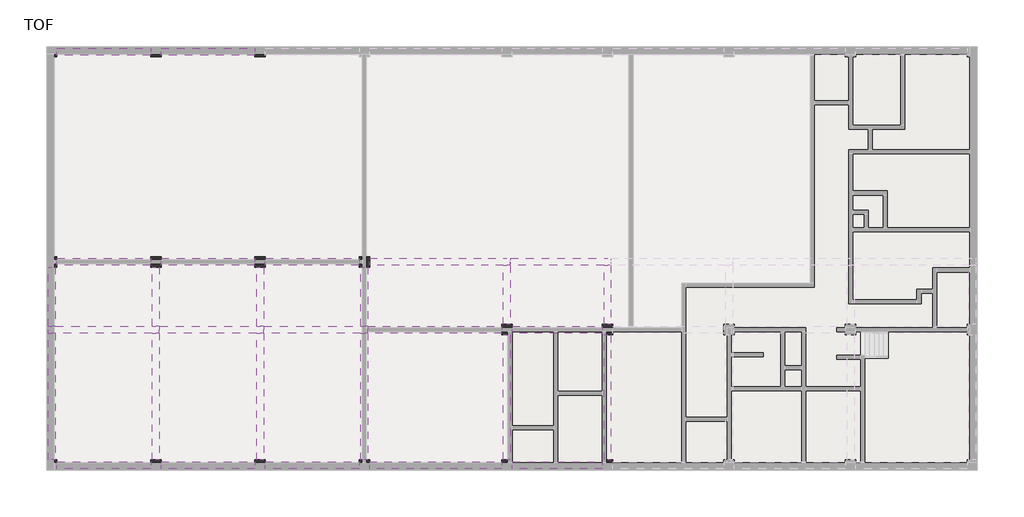
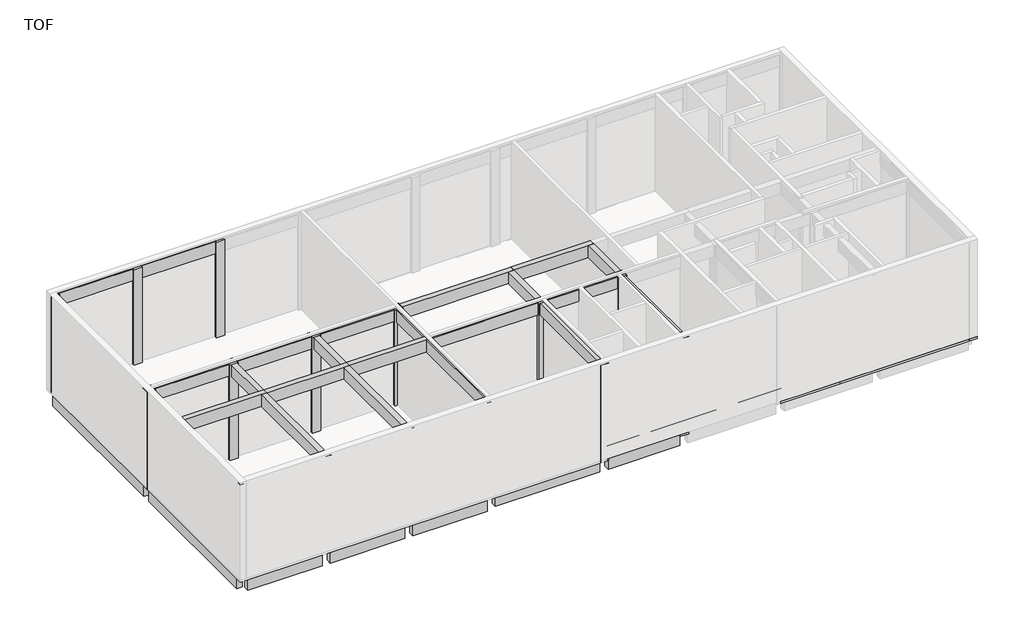
# One storey, part 2 of 3: 38 beams, 15 columns, 4 slabs.
"""IFC4 building model written with IfcOpenShell, lengths in millimetres."""

from ifc_helpers import new_model, si_unit, frame, origin, origin_with_axes, place, context, project, spatial, polyline, outline, extrude, faceted_brep, element, save

model = new_model("IFC4")

# Units and contexts
model_context = context("Model", 3, world=origin())
ifc_project = project(units=[si_unit("LENGTHUNIT", "METRE", prefix="MILLI")], contexts=[model_context])

# Site, building, storey
site = spatial("IfcSite", under=ifc_project)
building = spatial("IfcBuilding", under=site)
storey = spatial("IfcBuildingStorey", under=building, Name="TOF", Elevation=150.0)

# Beams
placement = place(None, origin())
element("IfcBeam", 1, ObjectType="RC Beam_Rectangular : H_SB_ACB_B400xH900", at=placement, inside=storey, context=model_context, shape_type="SweptSolid", body=[
    extrude(outline(polyline([(124.7, 12616.5208589), (-275.3, 12616.5208589), (-275.3, 24116.5208589), (124.7, 24116.5208589), (124.7, 12616.5208589)])), frame((0.0, 0.0, -900.0), z_axis=(0.0, 0.0, 1.0), x_axis=(1.0, 0.0, 0.0)), (0.0, 0.0, 1.0), 900.0),
])
element("IfcBeam", 2, ObjectType="RC Beam_Rectangular : H_SB_ACB_B400xH900", at=placement, inside=storey, context=model_context, shape_type="SweptSolid", body=[
    extrude(outline(polyline([(124.7, 916.5208589), (-275.3, 916.5208589), (-275.3, 12016.5208589), (124.7, 12016.5208589), (124.7, 916.5208589)])), frame((0.0, 0.0, -900.0), z_axis=(0.0, 0.0, 1.0), x_axis=(1.0, 0.0, 0.0)), (0.0, 0.0, 1.0), 900.0),
])
element("IfcBeam", 3, ObjectType="RC Beam_Rectangular : H_SB_ACB_B400xH900", at=placement, inside=storey, context=model_context, shape_type="SweptSolid", body=[
    extrude(outline(polyline([(5624.7, 24616.5208589), (5624.7, 24216.5208589), (224.7, 24216.5208589), (224.7, 24616.5208589), (5624.7, 24616.5208589)])), frame((0.0, 0.0, -900.0), z_axis=(0.0, 0.0, 1.0), x_axis=(1.0, 0.0, 0.0)), (0.0, 0.0, 1.0), 900.0),
])
element("IfcBeam", 4, ObjectType="RC Beam_Rectangular : H_SB_ACB_B400xH900", at=placement, inside=storey, context=model_context, shape_type="SweptSolid", body=[
    extrude(outline(polyline([(6224.7, 24216.5208589), (6224.7, 24616.5208589), (11624.7, 24616.5208589), (11624.7, 24216.5208589), (6224.7, 24216.5208589)])), frame((0.0, 0.0, -900.0), z_axis=(0.0, 0.0, 1.0), x_axis=(1.0, 0.0, 0.0)), (0.0, 0.0, 1.0), 900.0),
])
element("IfcBeam", 5, ObjectType="RC Beam_Rectangular : H_SB_ACB_B400xH900", at=placement, inside=storey, context=model_context, shape_type="SweptSolid", body=[
    extrude(outline(polyline([(224.7, 416.5208589), (224.7, 816.5208589), (5624.7, 816.5208589), (5624.7, 416.5208589), (224.7, 416.5208589)])), frame((0.0, 0.0, -900.0), z_axis=(0.0, 0.0, 1.0), x_axis=(1.0, 0.0, 0.0)), (0.0, 0.0, 1.0), 900.0),
])
element("IfcBeam", 6, ObjectType="RC Beam_Rectangular : H_SB_ACB_B400xH900", at=placement, inside=storey, context=model_context, shape_type="SweptSolid", body=[
    extrude(outline(polyline([(6224.7, 416.5208589), (6224.7, 816.5208589), (11624.7, 816.5208589), (11624.7, 416.5208589), (6224.7, 416.5208589)])), frame((0.0, 0.0, -900.0), z_axis=(0.0, 0.0, 1.0), x_axis=(1.0, 0.0, 0.0)), (0.0, 0.0, 1.0), 900.0),
])
element("IfcBeam", 7, ObjectType="RC Beam_Rectangular : H_SB_ACB_B400xH900", at=placement, inside=storey, context=model_context, shape_type="SweptSolid", body=[
    extrude(outline(polyline([(12224.7, 416.5208589), (12224.7, 816.5208589), (17624.7, 816.5208589), (17624.7, 416.5208589), (12224.7, 416.5208589)])), frame((0.0, 0.0, -900.0), z_axis=(0.0, 0.0, 1.0), x_axis=(1.0, 0.0, 0.0)), (0.0, 0.0, 1.0), 900.0),
])
element("IfcBeam", 8, ObjectType="RC Beam_Rectangular : H_SB_ACB_B400xH900", at=placement, inside=storey, context=model_context, shape_type="SweptSolid", body=[
    extrude(outline(polyline([(18224.7, 416.5208589), (18224.7, 816.5208589), (25824.7, 816.5208589), (25824.7, 416.5208589), (18224.7, 416.5208589)])), frame((0.0, 0.0, -750.0), z_axis=(0.0, 0.0, 1.0), x_axis=(1.0, 0.0, 0.0)), (0.0, 0.0, 1.0), 900.0),
])
element("IfcBeam", 9, ObjectType="RC Beam_Rectangular : H_SB_ACB_B400xH900", at=placement, inside=storey, context=model_context, shape_type="SweptSolid", body=[
    extrude(outline(polyline([(26424.7, 416.5208589), (26424.7, 816.5208589), (31624.7, 816.5208589), (31624.7, 416.5208589), (26424.7, 416.5208589)])), frame((0.0, 0.0, -750.0), z_axis=(0.0, 0.0, 1.0), x_axis=(1.0, 0.0, 0.0)), (0.0, 0.0, 1.0), 900.0),
])
element("IfcBeam", 10, ObjectType="RC Beam_Rectangular : H_SB_ACB_B400xH900", at=placement, inside=storey, context=model_context, shape_type="SweptSolid", body=[
    extrude(outline(polyline([(224.7, 12116.5208589), (224.7, 12516.5208589), (5624.7, 12516.5208589), (5624.7, 12116.5208589), (224.7, 12116.5208589)])), frame((0.0, 0.0, 6600.0), z_axis=(0.0, 0.0, 1.0), x_axis=(1.0, 0.0, 0.0)), (0.0, 0.0, 1.0), 900.0),
])
element("IfcBeam", 11, ObjectType="RC Beam_Rectangular : H_SB_ACB_B400xH900", at=placement, inside=storey, context=model_context, shape_type="SweptSolid", body=[
    extrude(outline(polyline([(6224.7, 12116.5208589), (6224.7, 12516.5208589), (11624.7, 12516.5208589), (11624.7, 12116.5208589), (6224.7, 12116.5208589)])), frame((0.0, 0.0, 6600.0), z_axis=(0.0, 0.0, 1.0), x_axis=(1.0, 0.0, 0.0)), (0.0, 0.0, 1.0), 900.0),
])
element("IfcBeam", 12, ObjectType="RC Beam_Rectangular : H_SB_ACB_B400xH900", at=placement, inside=storey, context=model_context, shape_type="SweptSolid", body=[
    extrude(outline(polyline([(12224.7, 12116.5208589), (12224.7, 12516.5208589), (17624.7, 12516.5208589), (17624.7, 12116.5208589), (12224.7, 12116.5208589)])), frame((0.0, 0.0, 6600.0), z_axis=(0.0, 0.0, 1.0), x_axis=(1.0, 0.0, 0.0)), (0.0, 0.0, 1.0), 900.0),
])
element("IfcBeam", 13, ObjectType="RC Beam_Rectangular : H_SB_ACB_B400xH900", at=placement, inside=storey, context=model_context, shape_type="Brep", body=[
    faceted_brep([(26324.7, 12116.5208589, 7500.0), (26324.7, 12303.8208589, 7500.0), (26324.7, 12516.5208589, 7500.0), (25924.7, 12516.5208589, 7500.0), (18224.7, 12516.5208589, 7500.0), (18224.7, 12116.5208589, 7500.0), (25924.7, 12116.5208589, 7500.0), (26324.7, 12116.5208589, 6600.0), (18224.7, 12116.5208589, 6600.0), (25924.7, 12116.5208589, 6600.0), (26324.7, 12516.5208589, 6600.0), (18224.7, 12516.5208589, 6600.0), (26324.7, 12516.5208589, 6750.0)], [[[0, 1, 2, 3, 4, 5, 6]], [[7, 0, 6, 5, 8, 9]], [[10, 7, 9, 8, 11]], [[2, 12, 10, 11, 4, 3]], [[5, 4, 11, 8]], [[2, 1, 0, 7, 10, 12]]]),
])
element("IfcBeam", 14, ObjectType="RC Beam_Rectangular : H_SB_ACB_B400xH900", at=placement, inside=storey, context=model_context, shape_type="Brep", body=[
    faceted_brep([(32124.7, 12116.5208589, 7500.0), (32124.7, 12303.8208589, 7500.0), (32124.7, 12516.5208589, 7500.0), (31724.7, 12516.5208589, 7500.0), (26324.7, 12516.5208589, 7500.0), (26324.7, 12116.5208589, 7500.0), (31724.7, 12116.5208589, 7500.0), (32124.7, 12116.5208589, 6600.0), (26324.7, 12116.5208589, 6600.0), (31724.7, 12116.5208589, 6600.0), (32124.7, 12516.5208589, 6600.0), (26324.7, 12516.5208589, 6600.0), (32124.7, 12516.5208589, 6750.0)], [[[0, 1, 2, 3, 4, 5, 6]], [[7, 0, 6, 5, 8, 9]], [[10, 7, 9, 8, 11]], [[2, 12, 10, 11, 4, 3]], [[2, 1, 0, 7, 10, 12]], [[5, 4, 11, 8]]]),
])
element("IfcBeam", 15, ObjectType="RC Beam_Rectangular : H_SB_ACB_B400xH900", at=placement, inside=storey, context=model_context, shape_type="SweptSolid", body=[
    extrude(outline(polyline([(224.7, 24216.5208589), (224.7, 24616.5208589), (5624.7, 24616.5208589), (5624.7, 24216.5208589), (224.7, 24216.5208589)])), frame((0.0, 0.0, 6600.0), z_axis=(0.0, 0.0, 1.0), x_axis=(1.0, 0.0, 0.0)), (0.0, 0.0, 1.0), 900.0),
])
element("IfcBeam", 16, ObjectType="RC Beam_Rectangular : H_SB_ACB_B400xH900", at=placement, inside=storey, context=model_context, shape_type="SweptSolid", body=[
    extrude(outline(polyline([(6224.7, 24216.5208589), (6224.7, 24616.5208589), (11624.7, 24616.5208589), (11624.7, 24216.5208589), (6224.7, 24216.5208589)])), frame((0.0, 0.0, 6600.0), z_axis=(0.0, 0.0, 1.0), x_axis=(1.0, 0.0, 0.0)), (0.0, 0.0, 1.0), 900.0),
])
element("IfcBeam", 17, ObjectType="RC Beam_Rectangular : H_SB_ACB_B400xH900", at=placement, inside=storey, context=model_context, shape_type="Brep", body=[
    faceted_brep([(-275.3, 8616.5208589, 7500.0), (-275.3, 8216.5208589, 7500.0), (124.7, 8216.5208589, 7500.0), (5724.7, 8216.5208589, 7500.0), (6124.7, 8216.5208589, 7500.0), (6124.7, 8616.5208589, 7500.0), (5724.7, 8616.5208589, 7500.0), (124.7, 8616.5208589, 7500.0), (-275.3, 8216.5208589, 6600.0), (124.7, 8216.5208589, 6600.0), (5724.7, 8216.5208589, 6600.0), (6124.7, 8216.5208589, 6600.0), (-275.3, 8616.5208589, 6600.0), (124.7, 8616.5208589, 6600.0), (5724.7, 8616.5208589, 6600.0), (6124.7, 8616.5208589, 6600.0)], [[[0, 1, 2, 3, 4, 5, 6, 7]], [[1, 8, 9, 10, 11, 4, 3, 2]], [[8, 12, 13, 14, 15, 11, 10, 9]], [[12, 0, 7, 6, 5, 15, 14, 13]], [[1, 0, 12, 8]], [[5, 4, 11, 15]]]),
])
element("IfcBeam", 18, ObjectType="RC Beam_Rectangular : H_SB_ACB_B400xH900", at=placement, inside=storey, context=model_context, shape_type="Brep", body=[
    faceted_brep([(12124.7, 8216.5208589, 7500.0), (12124.7, 8616.5208589, 7500.0), (11724.7, 8616.5208589, 7500.0), (6124.7, 8616.5208589, 7500.0), (6124.7, 8216.5208589, 7500.0), (11724.7, 8216.5208589, 7500.0), (12124.7, 8216.5208589, 6600.0), (6124.7, 8216.5208589, 6600.0), (11724.7, 8216.5208589, 6600.0), (12124.7, 8616.5208589, 6600.0), (6124.7, 8616.5208589, 6600.0), (11724.7, 8616.5208589, 6600.0)], [[[0, 1, 2, 3, 4, 5]], [[6, 0, 5, 4, 7, 8]], [[9, 6, 8, 7, 10, 11]], [[1, 9, 11, 10, 3, 2]], [[1, 0, 6, 9]], [[4, 3, 10, 7]]]),
])
element("IfcBeam", 19, ObjectType="RC Beam_Rectangular : H_SB_ACB_B400xH900", at=placement, inside=storey, context=model_context, shape_type="Brep", body=[
    faceted_brep([(18124.7, 8216.5208589, 7500.0), (18124.7, 8616.5208589, 7500.0), (17724.7, 8616.5208589, 7500.0), (12124.7, 8616.5208589, 7500.0), (12124.7, 8216.5208589, 7500.0), (17724.7, 8216.5208589, 7500.0), (18124.7, 8216.5208589, 6600.0), (12124.7, 8216.5208589, 6600.0), (17724.7, 8216.5208589, 6600.0), (18124.7, 8616.5208589, 6600.0), (12124.7, 8616.5208589, 6600.0), (17724.7, 8616.5208589, 6600.0)], [[[0, 1, 2, 3, 4, 5]], [[6, 0, 5, 4, 7, 8]], [[9, 6, 8, 7, 10, 11]], [[1, 9, 11, 10, 3, 2]], [[1, 0, 6, 9]], [[4, 3, 10, 7]]]),
])
element("IfcBeam", 20, ObjectType="RC Beam_Rectangular : H_SB_ACB_B400xH900", at=placement, inside=storey, context=model_context, shape_type="SweptSolid", body=[
    extrude(outline(polyline([(18124.7, 8216.5208589), (18124.7, 8616.5208589), (25824.7, 8616.5208589), (25824.7, 8216.5208589), (18124.7, 8216.5208589)])), frame((0.0, 0.0, 6600.0), z_axis=(0.0, 0.0, 1.0), x_axis=(1.0, 0.0, 0.0)), (0.0, 0.0, 1.0), 900.0),
])
element("IfcBeam", 21, ObjectType="RC Beam_Rectangular : H_SB_ACB_B400xH900", at=placement, inside=storey, context=model_context, shape_type="SweptSolid", body=[
    extrude(outline(polyline([(26424.7, 8216.5208589), (26424.7, 8616.5208589), (31624.7, 8616.5208589), (31624.7, 8216.5208589), (26424.7, 8216.5208589)])), frame((0.0, 0.0, 6600.0), z_axis=(0.0, 0.0, 1.0), x_axis=(1.0, 0.0, 0.0)), (0.0, 0.0, 1.0), 900.0),
])
element("IfcBeam", 22, ObjectType="RC Beam_Rectangular : H_SB_ACB_B400xH900", at=placement, inside=storey, context=model_context, shape_type="SweptSolid", body=[
    extrude(outline(polyline([(224.7, 416.5208589), (224.7, 816.5208589), (5624.7, 816.5208589), (5624.7, 416.5208589), (224.7, 416.5208589)])), frame((0.0, 0.0, 6600.0), z_axis=(0.0, 0.0, 1.0), x_axis=(1.0, 0.0, 0.0)), (0.0, 0.0, 1.0), 900.0),
])
element("IfcBeam", 23, ObjectType="RC Beam_Rectangular : H_SB_ACB_B400xH900", at=placement, inside=storey, context=model_context, shape_type="SweptSolid", body=[
    extrude(outline(polyline([(6224.7, 416.5208589), (6224.7, 816.5208589), (11624.7, 816.5208589), (11624.7, 416.5208589), (6224.7, 416.5208589)])), frame((0.0, 0.0, 6600.0), z_axis=(0.0, 0.0, 1.0), x_axis=(1.0, 0.0, 0.0)), (0.0, 0.0, 1.0), 900.0),
])
element("IfcBeam", 24, ObjectType="RC Beam_Rectangular : H_SB_ACB_B400xH900", at=placement, inside=storey, context=model_context, shape_type="SweptSolid", body=[
    extrude(outline(polyline([(12224.7, 416.5208589), (12224.7, 816.5208589), (17624.7, 816.5208589), (17624.7, 416.5208589), (12224.7, 416.5208589)])), frame((0.0, 0.0, 6600.0), z_axis=(0.0, 0.0, 1.0), x_axis=(1.0, 0.0, 0.0)), (0.0, 0.0, 1.0), 900.0),
])
element("IfcBeam", 25, ObjectType="RC Beam_Rectangular : H_SB_ACB_B400xH900", at=placement, inside=storey, context=model_context, shape_type="SweptSolid", body=[
    extrude(outline(polyline([(18224.7, 416.5208589), (18224.7, 816.5208589), (25824.7, 816.5208589), (25824.7, 416.5208589), (18224.7, 416.5208589)])), frame((0.0, 0.0, 6600.0), z_axis=(0.0, 0.0, 1.0), x_axis=(1.0, 0.0, 0.0)), (0.0, 0.0, 1.0), 900.0),
])
element("IfcBeam", 26, ObjectType="RC Beam_Rectangular : H_SB_ACB_B400xH900", at=placement, inside=storey, context=model_context, shape_type="SweptSolid", body=[
    extrude(outline(polyline([(26424.7, 416.5208589), (26424.7, 816.5208589), (31624.7, 816.5208589), (31624.7, 416.5208589), (26424.7, 416.5208589)])), frame((0.0, 0.0, 6600.0), z_axis=(0.0, 0.0, 1.0), x_axis=(1.0, 0.0, 0.0)), (0.0, 0.0, 1.0), 900.0),
])
element("IfcBeam", 27, ObjectType="RC Beam_Rectangular : H_SB_ACB_B400xH900", at=placement, inside=storey, context=model_context, shape_type="SweptSolid", body=[
    extrude(outline(polyline([(-275.3, 8216.5208589), (124.7, 8216.5208589), (124.7, 916.5208589), (-275.3, 916.5208589), (-275.3, 8216.5208589)])), frame((0.0, 0.0, 6600.0), z_axis=(0.0, 0.0, 1.0), x_axis=(1.0, 0.0, 0.0)), (0.0, 0.0, 1.0), 900.0),
])
element("IfcBeam", 28, ObjectType="RC Beam_Rectangular : H_SB_ACB_B400xH900", at=placement, inside=storey, context=model_context, shape_type="SweptSolid", body=[
    extrude(outline(polyline([(124.7, 8616.5208589), (-275.3, 8616.5208589), (-275.3, 12016.5208589), (124.7, 12016.5208589), (124.7, 8616.5208589)])), frame((0.0, 0.0, 6600.0), z_axis=(0.0, 0.0, 1.0), x_axis=(1.0, 0.0, 0.0)), (0.0, 0.0, 1.0), 900.0),
])
element("IfcBeam", 29, ObjectType="RC Beam_Rectangular : H_SB_ACB_B400xH900", at=placement, inside=storey, context=model_context, shape_type="SweptSolid", body=[
    extrude(outline(polyline([(5724.7, 8216.5208589), (6124.7, 8216.5208589), (6124.7, 916.5208589), (5724.7, 916.5208589), (5724.7, 8216.5208589)])), frame((0.0, 0.0, 6600.0), z_axis=(0.0, 0.0, 1.0), x_axis=(1.0, 0.0, 0.0)), (0.0, 0.0, 1.0), 900.0),
])
element("IfcBeam", 30, ObjectType="RC Beam_Rectangular : H_SB_ACB_B400xH900", at=placement, inside=storey, context=model_context, shape_type="SweptSolid", body=[
    extrude(outline(polyline([(6124.7, 8616.5208589), (5724.7, 8616.5208589), (5724.7, 12016.5208589), (6124.7, 12016.5208589), (6124.7, 8616.5208589)])), frame((0.0, 0.0, 6600.0), z_axis=(0.0, 0.0, 1.0), x_axis=(1.0, 0.0, 0.0)), (0.0, 0.0, 1.0), 900.0),
])
element("IfcBeam", 31, ObjectType="RC Beam_Rectangular : H_SB_ACB_B400xH900", at=placement, inside=storey, context=model_context, shape_type="SweptSolid", body=[
    extrude(outline(polyline([(11724.7, 8216.5208589), (12124.7, 8216.5208589), (12124.7, 916.5208589), (11724.7, 916.5208589), (11724.7, 8216.5208589)])), frame((0.0, 0.0, 6600.0), z_axis=(0.0, 0.0, 1.0), x_axis=(1.0, 0.0, 0.0)), (0.0, 0.0, 1.0), 900.0),
])
element("IfcBeam", 32, ObjectType="RC Beam_Rectangular : H_SB_ACB_B400xH900", at=placement, inside=storey, context=model_context, shape_type="SweptSolid", body=[
    extrude(outline(polyline([(12124.7, 8616.5208589), (11724.7, 8616.5208589), (11724.7, 12016.5208589), (12124.7, 12016.5208589), (12124.7, 8616.5208589)])), frame((0.0, 0.0, 6600.0), z_axis=(0.0, 0.0, 1.0), x_axis=(1.0, 0.0, 0.0)), (0.0, 0.0, 1.0), 900.0),
])
element("IfcBeam", 33, ObjectType="RC Beam_Rectangular : H_SB_ACB_B400xH900", at=placement, inside=storey, context=model_context, shape_type="SweptSolid", body=[
    extrude(outline(polyline([(17724.7, 8216.5208589), (18124.7, 8216.5208589), (18124.7, 916.5208589), (17724.7, 916.5208589), (17724.7, 8216.5208589)])), frame((0.0, 0.0, 6600.0), z_axis=(0.0, 0.0, 1.0), x_axis=(1.0, 0.0, 0.0)), (0.0, 0.0, 1.0), 900.0),
])
element("IfcBeam", 34, ObjectType="RC Beam_Rectangular : H_SB_ACB_B400xH900", at=placement, inside=storey, context=model_context, shape_type="SweptSolid", body=[
    extrude(outline(polyline([(18124.7, 8616.5208589), (17724.7, 8616.5208589), (17724.7, 12016.5208589), (18124.7, 12016.5208589), (18124.7, 8616.5208589)])), frame((0.0, 0.0, 6600.0), z_axis=(0.0, 0.0, 1.0), x_axis=(1.0, 0.0, 0.0)), (0.0, 0.0, 1.0), 900.0),
])
element("IfcBeam", 35, ObjectType="RC Beam_Rectangular : H_SB_ACB_B400xH900", at=placement, inside=storey, context=model_context, shape_type="SweptSolid", body=[
    extrude(outline(polyline([(25924.7, 8116.5208589), (26324.7, 8116.5208589), (26324.7, 916.5208589), (25924.7, 916.5208589), (25924.7, 8116.5208589)])), frame((0.0, 0.0, 6600.0), z_axis=(0.0, 0.0, 1.0), x_axis=(1.0, 0.0, 0.0)), (0.0, 0.0, 1.0), 900.0),
])
element("IfcBeam", 36, ObjectType="RC Beam_Rectangular : H_SB_ACB_B400xH900", at=placement, inside=storey, context=model_context, shape_type="SweptSolid", body=[
    extrude(outline(polyline([(25924.7, 12116.5208589), (26324.7, 12116.5208589), (26324.7, 8716.5208589), (25924.7, 8716.5208589), (25924.7, 12116.5208589)])), frame((0.0, 0.0, 6600.0), z_axis=(0.0, 0.0, 1.0), x_axis=(1.0, 0.0, 0.0)), (0.0, 0.0, 1.0), 900.0),
])
element("IfcBeam", 37, ObjectType="RC Beam_Rectangular : H_SB_ACB_B400xH900", at=placement, inside=storey, context=model_context, shape_type="SweptSolid", body=[
    extrude(outline(polyline([(31724.7, 8116.5208589), (32124.7, 8116.5208589), (32124.7, 916.5208589), (31724.7, 916.5208589), (31724.7, 8116.5208589)])), frame((0.0, 0.0, 6600.0), z_axis=(0.0, 0.0, 1.0), x_axis=(1.0, 0.0, 0.0)), (0.0, 0.0, 1.0), 900.0),
])
element("IfcBeam", 38, ObjectType="RC Beam_Rectangular : H_SB_ACB_B400xH900", at=placement, inside=storey, context=model_context, shape_type="SweptSolid", body=[
    extrude(outline(polyline([(31724.7, 12116.5208589), (32124.7, 12116.5208589), (32124.7, 8716.5208589), (31724.7, 8716.5208589), (31724.7, 12116.5208589)])), frame((0.0, 0.0, 6600.0), z_axis=(0.0, 0.0, 1.0), x_axis=(1.0, 0.0, 0.0)), (0.0, 0.0, 1.0), 900.0),
])

# Columns
element("IfcColumn", 39, ObjectType="RC_Column_Rectangular : H_SC_ACC_W600xL600", at=placement, inside=storey, context=model_context, shape_type="Brep", body=[
    faceted_brep([(224.7, 12016.5208589, 0.0), (-375.3, 12016.5208589, 0.0), (-375.3, 12316.5208589, 0.0), (224.7, 12316.5208589, 0.0), (224.7, 12616.5208589, 7500.0), (224.7, 12516.5208589, 7500.0), (224.7, 12116.5208589, 7500.0), (224.7, 12016.5208589, 7500.0), (224.7, 12316.5208589, 150.0), (224.7, 12616.5208589, 150.0), (124.7, 12016.5208589, 7500.0), (-275.3, 12016.5208589, 7500.0), (-375.3, 12016.5208589, 7500.0), (-375.3, 12616.5208589, 7500.0), (-375.3, 12616.5208589, 150.0), (-375.3, 12316.5208589, 150.0), (-275.3, 12616.5208589, 7500.0), (124.7, 12616.5208589, 7500.0)], [[[0, 1, 2, 3]], [[4, 5, 6, 7, 0, 3, 8, 9]], [[1, 0, 7, 10, 11, 12]], [[1, 12, 13, 14, 15, 2]], [[13, 16, 17, 4, 9, 14]], [[7, 6, 5, 4, 17, 16, 13, 12, 11, 10]], [[8, 15, 14, 9]], [[15, 8, 3, 2]]]),
])
element("IfcColumn", 40, ObjectType="RC_Column_Rectangular : H_SC_ACC_W600xL600", at=placement, inside=storey, context=model_context, shape_type="Brep", body=[
    faceted_brep([(6224.7, 12016.5208589, 0.0), (5624.7, 12016.5208589, 0.0), (5624.7, 12316.5208589, 0.0), (6224.7, 12316.5208589, 0.0), (6224.7, 12616.5208589, 7500.0), (6224.7, 12516.5208589, 7500.0), (6224.7, 12116.5208589, 7500.0), (6224.7, 12016.5208589, 7500.0), (6224.7, 12316.5208589, 150.0), (6224.7, 12616.5208589, 150.0), (6124.7, 12016.5208589, 7500.0), (5724.7, 12016.5208589, 7500.0), (5624.7, 12016.5208589, 7500.0), (5624.7, 12116.5208589, 7500.0), (5624.7, 12516.5208589, 7500.0), (5624.7, 12616.5208589, 7500.0), (5624.7, 12616.5208589, 150.0), (5624.7, 12316.5208589, 150.0), (5724.7, 12616.5208589, 7500.0), (6124.7, 12616.5208589, 7500.0)], [[[0, 1, 2, 3]], [[4, 5, 6, 7, 0, 3, 8, 9]], [[1, 0, 7, 10, 11, 12]], [[1, 12, 13, 14, 15, 16, 17, 2]], [[15, 18, 19, 4, 9, 16]], [[7, 6, 5, 4, 19, 18, 15, 14, 13, 12, 11, 10]], [[8, 17, 16, 9]], [[17, 8, 3, 2]]]),
])
element("IfcColumn", 41, ObjectType="RC_Column_Rectangular : H_SC_ACC_W600xL600", at=placement, inside=storey, context=model_context, shape_type="Brep", body=[
    faceted_brep([(12224.7, 12016.5208589, 0.0), (11624.7, 12016.5208589, 0.0), (11624.7, 12316.5208589, 0.0), (12224.7, 12316.5208589, 0.0), (12224.7, 12616.5208589, 7500.0), (12224.7, 12516.5208589, 7500.0), (12224.7, 12116.5208589, 7500.0), (12224.7, 12016.5208589, 7500.0), (12224.7, 12316.5208589, 150.0), (12224.7, 12616.5208589, 150.0), (12124.7, 12016.5208589, 7500.0), (11724.7, 12016.5208589, 7500.0), (11624.7, 12016.5208589, 7500.0), (11624.7, 12116.5208589, 7500.0), (11624.7, 12516.5208589, 7500.0), (11624.7, 12616.5208589, 7500.0), (11624.7, 12616.5208589, 150.0), (11624.7, 12316.5208589, 150.0), (11724.7, 12616.5208589, 7500.0), (12124.7, 12616.5208589, 7500.0)], [[[0, 1, 2, 3]], [[4, 5, 6, 7, 0, 3, 8, 9]], [[1, 0, 7, 10, 11, 12]], [[1, 12, 13, 14, 15, 16, 17, 2]], [[15, 18, 19, 4, 9, 16]], [[7, 6, 5, 4, 19, 18, 15, 14, 13, 12, 11, 10]], [[8, 17, 16, 9]], [[17, 8, 3, 2]]]),
])
element("IfcColumn", 42, ObjectType="RC_Column_Rectangular : H_SC_ACC_W600xL600", at=placement, inside=storey, context=model_context, shape_type="Brep", body=[
    faceted_brep([(17924.7, 12016.5208589, 0.0), (17624.7, 12016.5208589, 0.0), (17624.7, 12316.5208589, 0.0), (17924.7, 12316.5208589, 0.0), (18224.7, 12616.5208589, 7500.0), (18224.7, 12516.5208589, 7500.0), (18224.7, 12116.5208589, 7500.0), (18224.7, 12016.5208589, 7500.0), (18224.7, 12016.5208589, 150.0), (18224.7, 12616.5208589, 150.0), (18124.7, 12016.5208589, 7500.0), (17724.7, 12016.5208589, 7500.0), (17624.7, 12016.5208589, 7500.0), (17924.7, 12016.5208589, 150.0), (17624.7, 12116.5208589, 7500.0), (17624.7, 12516.5208589, 7500.0), (17624.7, 12616.5208589, 7500.0), (17624.7, 12616.5208589, 150.0), (17624.7, 12316.5208589, 150.0), (17724.7, 12616.5208589, 7500.0), (18124.7, 12616.5208589, 7500.0), (17924.7, 12316.5208589, 150.0)], [[[0, 1, 2, 3]], [[4, 5, 6, 7, 8, 9]], [[7, 10, 11, 12, 1, 0, 13, 8]], [[1, 12, 14, 15, 16, 17, 18, 2]], [[16, 19, 20, 4, 9, 17]], [[7, 6, 5, 4, 20, 19, 16, 15, 14, 12, 11, 10]], [[13, 21, 18, 17, 9, 8]], [[3, 21, 13, 0]], [[21, 3, 2, 18]]]),
])
element("IfcColumn", 43, ObjectType="RC_Column_Rectangular : H_SC_ACC_W600xL600", at=placement, inside=storey, context=model_context, shape_type="Brep", body=[
    faceted_brep([(224.7, 24716.5208589, 7500.0), (224.7, 24616.5208589, 7500.0), (224.7, 24216.5208589, 7500.0), (224.7, 24116.5208589, 7500.0), (224.7, 24116.5208589, 150.0), (224.7, 24716.5208589, 150.0), (124.7, 24116.5208589, 7500.0), (-275.3, 24116.5208589, 7500.0), (-375.3, 24116.5208589, 7500.0), (-375.3, 24116.5208589, 150.0), (-375.3, 24716.5208589, 7500.0), (-375.3, 24716.5208589, 150.0)], [[[0, 1, 2, 3, 4, 5]], [[3, 6, 7, 8, 9, 4]], [[8, 10, 11, 9]], [[10, 0, 5, 11]], [[3, 2, 1, 0, 10, 8, 7, 6]], [[5, 4, 9, 11]]]),
])
element("IfcColumn", 44, ObjectType="RC_Column_Rectangular : H_SC_ACC_W600xL600", at=placement, inside=storey, context=model_context, shape_type="Brep", body=[
    faceted_brep([(6224.7, 24716.5208589, 7500.0), (6224.7, 24616.5208589, 7500.0), (6224.7, 24216.5208589, 7500.0), (6224.7, 24116.5208589, 7500.0), (6224.7, 24116.5208589, 150.0), (6224.7, 24716.5208589, 150.0), (6124.7, 24116.5208589, 7500.0), (5724.7, 24116.5208589, 7500.0), (5624.7, 24116.5208589, 7500.0), (5624.7, 24116.5208589, 150.0), (5624.7, 24216.5208589, 7500.0), (5624.7, 24616.5208589, 7500.0), (5624.7, 24716.5208589, 7500.0), (5624.7, 24716.5208589, 150.0)], [[[0, 1, 2, 3, 4, 5]], [[3, 6, 7, 8, 9, 4]], [[8, 10, 11, 12, 13, 9]], [[12, 0, 5, 13]], [[3, 2, 1, 0, 12, 11, 10, 8, 7, 6]], [[5, 4, 9, 13]]]),
])
element("IfcColumn", 45, ObjectType="RC_Column_Rectangular : H_SC_ACC_W600xL600", at=placement, inside=storey, context=model_context, shape_type="Brep", body=[
    faceted_brep([(12224.7, 24716.5208589, 7500.0), (12224.7, 24616.5208589, 7500.0), (12224.7, 24216.5208589, 7500.0), (12224.7, 24116.5208589, 7500.0), (12224.7, 24116.5208589, 150.0), (12224.7, 24716.5208589, 150.0), (12124.7, 24116.5208589, 7500.0), (11724.7, 24116.5208589, 7500.0), (11624.7, 24116.5208589, 7500.0), (11624.7, 24116.5208589, 150.0), (11624.7, 24216.5208589, 7500.0), (11624.7, 24616.5208589, 7500.0), (11624.7, 24716.5208589, 7500.0), (11624.7, 24716.5208589, 150.0)], [[[0, 1, 2, 3, 4, 5]], [[3, 6, 7, 8, 9, 4]], [[8, 10, 11, 12, 13, 9]], [[12, 0, 5, 13]], [[3, 2, 1, 0, 12, 11, 10, 8, 7, 6]], [[5, 4, 9, 13]]]),
])
element("IfcColumn", 46, ObjectType="RC_Column_Rectangular : H_SC_ACC_W600xL600", at=placement, inside=storey, context=model_context, shape_type="Brep", body=[
    faceted_brep([(26424.7, 8116.5208589, 0.0), (25824.7, 8116.5208589, 0.0), (25824.7, 8416.5208589, 0.0), (26424.7, 8416.5208589, 0.0), (26424.7, 8716.5208589, 7500.0), (26424.7, 8616.5208589, 7500.0), (26424.7, 8216.5208589, 7500.0), (26424.7, 8116.5208589, 7500.0), (26424.7, 8416.5208589, 150.0), (26424.7, 8716.5208589, 150.0), (26324.7, 8116.5208589, 7500.0), (25924.7, 8116.5208589, 7500.0), (25824.7, 8116.5208589, 7500.0), (25824.7, 8216.5208589, 7500.0), (25824.7, 8616.5208589, 7500.0), (25824.7, 8716.5208589, 7500.0), (25824.7, 8716.5208589, 150.0), (25824.7, 8416.5208589, 150.0), (25924.7, 8716.5208589, 7500.0), (26324.7, 8716.5208589, 7500.0)], [[[0, 1, 2, 3]], [[4, 5, 6, 7, 0, 3, 8, 9]], [[1, 0, 7, 10, 11, 12]], [[1, 12, 13, 14, 15, 16, 17, 2]], [[15, 18, 19, 4, 9, 16]], [[7, 6, 5, 4, 19, 18, 15, 14, 13, 12, 11, 10]], [[8, 17, 16, 9]], [[17, 8, 3, 2]]]),
])
element("IfcColumn", 47, ObjectType="RC_Column_Rectangular : H_SC_ACC_W600xL600", at=placement, inside=storey, context=model_context, shape_type="Brep", body=[
    faceted_brep([(32224.7, 8116.5208589, 0.0), (31624.7, 8116.5208589, 0.0), (31624.7, 8416.5208589, 0.0), (32224.7, 8416.5208589, 0.0), (32224.7, 8716.5208589, 7500.0), (32224.7, 8616.5208589, 7500.0), (32224.7, 8216.5208589, 7500.0), (32224.7, 8116.5208589, 7500.0), (32224.7, 8416.5208589, 150.0), (32224.7, 8716.5208589, 150.0), (32124.7, 8116.5208589, 7500.0), (31724.7, 8116.5208589, 7500.0), (31624.7, 8116.5208589, 7500.0), (31624.7, 8216.5208589, 7500.0), (31624.7, 8616.5208589, 7500.0), (31624.7, 8716.5208589, 7500.0), (31624.7, 8716.5208589, 150.0), (31624.7, 8416.5208589, 150.0), (31724.7, 8716.5208589, 7500.0), (32124.7, 8716.5208589, 7500.0)], [[[0, 1, 2, 3]], [[4, 5, 6, 7, 0, 3, 8, 9]], [[1, 0, 7, 10, 11, 12]], [[1, 12, 13, 14, 15, 16, 17, 2]], [[15, 18, 19, 4, 9, 16]], [[7, 6, 5, 4, 19, 18, 15, 14, 13, 12, 11, 10]], [[8, 17, 16, 9]], [[17, 8, 3, 2]]]),
])
element("IfcColumn", 48, ObjectType="RC_Column_Rectangular : H_SC_ACC_W600xL600", at=placement, inside=storey, context=model_context, shape_type="Brep", body=[
    faceted_brep([(224.7, 916.5208589, 0.0), (224.7, 316.5208589, 0.0), (-375.3, 316.5208589, 0.0), (-375.3, 916.5208589, 0.0), (224.7, 916.5208589, 7500.0), (224.7, 816.5208589, 7500.0), (224.7, 416.5208589, 7500.0), (224.7, 316.5208589, 7500.0), (-375.3, 316.5208589, 7500.0), (-375.3, 916.5208589, 7500.0), (-275.3, 916.5208589, 7500.0), (124.7, 916.5208589, 7500.0)], [[[0, 1, 2, 3]], [[4, 5, 6, 7, 1, 0]], [[7, 8, 2, 1]], [[8, 9, 3, 2]], [[9, 10, 11, 4, 0, 3]], [[4, 11, 10, 9, 8, 7, 6, 5]]]),
])
element("IfcColumn", 49, ObjectType="RC_Column_Rectangular : H_SC_ACC_W600xL600", at=placement, inside=storey, context=model_context, shape_type="Brep", body=[
    faceted_brep([(6224.7, 916.5208589, 0.0), (6224.7, 316.5208589, 0.0), (5624.7, 316.5208589, 0.0), (5624.7, 916.5208589, 0.0), (6224.7, 916.5208589, 7500.0), (6224.7, 816.5208589, 7500.0), (6224.7, 416.5208589, 7500.0), (6224.7, 316.5208589, 7500.0), (5624.7, 316.5208589, 7500.0), (5624.7, 416.5208589, 7500.0), (5624.7, 816.5208589, 7500.0), (5624.7, 916.5208589, 7500.0), (5724.7, 916.5208589, 7500.0), (6124.7, 916.5208589, 7500.0)], [[[0, 1, 2, 3]], [[4, 5, 6, 7, 1, 0]], [[7, 8, 2, 1]], [[8, 9, 10, 11, 3, 2]], [[11, 12, 13, 4, 0, 3]], [[4, 13, 12, 11, 10, 9, 8, 7, 6, 5]]]),
])
element("IfcColumn", 50, ObjectType="RC_Column_Rectangular : H_SC_ACC_W600xL600", at=placement, inside=storey, context=model_context, shape_type="Brep", body=[
    faceted_brep([(12224.7, 916.5208589, 0.0), (12224.7, 316.5208589, 0.0), (11624.7, 316.5208589, 0.0), (11624.7, 916.5208589, 0.0), (12224.7, 916.5208589, 7500.0), (12224.7, 816.5208589, 7500.0), (12224.7, 416.5208589, 7500.0), (12224.7, 316.5208589, 7500.0), (11624.7, 316.5208589, 7500.0), (11624.7, 416.5208589, 7500.0), (11624.7, 816.5208589, 7500.0), (11624.7, 916.5208589, 7500.0), (11724.7, 916.5208589, 7500.0), (12124.7, 916.5208589, 7500.0)], [[[0, 1, 2, 3]], [[4, 5, 6, 7, 1, 0]], [[7, 8, 2, 1]], [[8, 9, 10, 11, 3, 2]], [[11, 12, 13, 4, 0, 3]], [[4, 13, 12, 11, 10, 9, 8, 7, 6, 5]]]),
])
element("IfcColumn", 51, ObjectType="RC_Column_Rectangular : H_SC_ACC_W600xL600", at=placement, inside=storey, context=model_context, shape_type="Brep", body=[
    faceted_brep([(18224.7, 916.5208589, 0.0), (18224.7, 316.5208589, 0.0), (17624.7, 316.5208589, 0.0), (17624.7, 916.5208589, 0.0), (18224.7, 916.5208589, 7500.0), (18224.7, 816.5208589, 7500.0), (18224.7, 416.5208589, 7500.0), (18224.7, 316.5208589, 7500.0), (17624.7, 316.5208589, 7500.0), (17624.7, 416.5208589, 7500.0), (17624.7, 816.5208589, 7500.0), (17624.7, 916.5208589, 7500.0), (17724.7, 916.5208589, 7500.0), (18124.7, 916.5208589, 7500.0)], [[[0, 1, 2, 3]], [[4, 5, 6, 7, 1, 0]], [[7, 8, 2, 1]], [[8, 9, 10, 11, 3, 2]], [[11, 12, 13, 4, 0, 3]], [[4, 13, 12, 11, 10, 9, 8, 7, 6, 5]]]),
])
element("IfcColumn", 52, ObjectType="RC_Column_Rectangular : H_SC_ACC_W600xL600", at=placement, inside=storey, context=model_context, shape_type="Brep", body=[
    faceted_brep([(26424.7, 916.5208589, 0.0), (26424.7, 316.5208589, 0.0), (25824.7, 316.5208589, 0.0), (25824.7, 916.5208589, 0.0), (26424.7, 916.5208589, 7500.0), (26424.7, 816.5208589, 7500.0), (26424.7, 416.5208589, 7500.0), (26424.7, 316.5208589, 7500.0), (25824.7, 316.5208589, 7500.0), (25824.7, 416.5208589, 7500.0), (25824.7, 816.5208589, 7500.0), (25824.7, 916.5208589, 7500.0), (25924.7, 916.5208589, 7500.0), (26324.7, 916.5208589, 7500.0)], [[[0, 1, 2, 3]], [[4, 5, 6, 7, 1, 0]], [[7, 8, 2, 1]], [[8, 9, 10, 11, 3, 2]], [[11, 12, 13, 4, 0, 3]], [[4, 13, 12, 11, 10, 9, 8, 7, 6, 5]]]),
])
element("IfcColumn", 53, ObjectType="RC_Column_Rectangular : H_SC_ACC_W600xL600", at=placement, inside=storey, context=model_context, shape_type="Brep", body=[
    faceted_brep([(32224.7, 916.5208589, 0.0), (32224.7, 316.5208589, 0.0), (31624.7, 316.5208589, 0.0), (31624.7, 916.5208589, 0.0), (32224.7, 916.5208589, 7500.0), (32224.7, 816.5208589, 7500.0), (32224.7, 416.5208589, 7500.0), (32224.7, 316.5208589, 7500.0), (31624.7, 316.5208589, 7500.0), (31624.7, 416.5208589, 7500.0), (31624.7, 816.5208589, 7500.0), (31624.7, 916.5208589, 7500.0), (31724.7, 916.5208589, 7500.0), (32124.7, 916.5208589, 7500.0)], [[[0, 1, 2, 3]], [[4, 5, 6, 7, 1, 0]], [[7, 8, 2, 1]], [[8, 9, 10, 11, 3, 2]], [[11, 12, 13, 4, 0, 3]], [[4, 13, 12, 11, 10, 9, 8, 7, 6, 5]]]),
])

# Slabs
element("IfcSlab", 54, ObjectType="H_FL_AMF_RC Slab_T150", at=placement, inside=storey, context=model_context, shape_type="Brep", body=[
    faceted_brep([(53224.7, 11850.5208589, 1000.0), (50777.7, 11850.5208589, 1000.0), (50777.7, 8416.5208589, 1000.0), (46624.7, 8416.5208589, 1000.0), (46624.7, 5013.5208589, 1000.0), (43341.7, 5013.5208589, 1000.0), (43224.7, 5013.5208589, 1000.0), (43224.7, 8299.5208589, 1000.0), (43224.7, 8416.5208589, 1000.0), (39041.7, 8416.5208589, 1000.0), (38924.7, 8416.5208589, 1000.0), (38924.7, 746.5208589, 1000.0), (38924.7, 316.5208589, 1000.0), (26307.7, 316.5208589, 1000.0), (26307.7, 8416.5208589, 1000.0), (36324.7, 8416.5208589, 1000.0), (36324.7, 10966.5208589, 1000.0), (43724.7, 10966.5208589, 1000.0), (43724.7, 24716.5208589, 1000.0), (53224.7, 24716.5208589, 1000.0), (53224.7, 11850.5208589, 1150.0), (53224.7, 24716.5208589, 1150.0), (43724.7, 24716.5208589, 1150.0), (43724.7, 10966.5208589, 1150.0), (36324.7, 10966.5208589, 1150.0), (36324.7, 8416.5208589, 1150.0), (26307.7, 8416.5208589, 1150.0), (26307.7, 316.5208589, 1150.0), (38924.7, 316.5208589, 1150.0), (38924.7, 746.5208589, 1150.0), (38924.7, 8416.5208589, 1150.0), (39041.7, 8416.5208589, 1150.0), (43224.7, 8416.5208589, 1150.0), (43224.7, 8299.5208589, 1150.0), (43224.7, 5013.5208589, 1150.0), (43341.7, 5013.5208589, 1150.0), (46624.7, 5013.5208589, 1150.0), (46624.7, 8416.5208589, 1150.0), (50777.7, 8416.5208589, 1150.0), (50777.7, 11850.5208589, 1150.0)], [[[0, 1, 2, 3, 4, 5, 6, 7, 8, 9, 10, 11, 12, 13, 14, 15, 16, 17, 18, 19]], [[20, 21, 22, 23, 24, 25, 26, 27, 28, 29, 30, 31, 32, 33, 34, 35, 36, 37, 38, 39]], [[13, 12, 28, 27]], [[19, 18, 22, 21]], [[0, 19, 21, 20]], [[1, 0, 20, 39]], [[2, 1, 39, 38]], [[3, 2, 38, 37]], [[4, 3, 37, 36]], [[6, 5, 4, 36, 35, 34]], [[8, 7, 6, 34, 33, 32]], [[10, 9, 8, 32, 31, 30]], [[12, 11, 10, 30, 29, 28]], [[14, 13, 27, 26]], [[15, 14, 26, 25]], [[16, 15, 25, 24]], [[17, 16, 24, 23]], [[18, 17, 23, 22]]]),
])
element("IfcSlab", 55, ObjectType="H_FL_AMF_RC Slab_T150", at=placement, inside=storey, context=model_context, shape_type="SweptSolid", body=[
    extrude(outline(polyline([(53224.7, 11850.5208589), (53224.7, 8416.5208589), (50777.7, 8416.5208589), (50777.7, 11850.5208589), (53224.7, 11850.5208589)])), frame((0.0, 0.0, 1000.0), z_axis=(0.0, 0.0, 1.0), x_axis=(1.0, 0.0, 0.0)), (0.0, 0.0, 1.0), 150.0),
])
element("IfcSlab", 56, ObjectType="H_FL_AMF_RC Slab_T150", at=placement, inside=storey, context=model_context, shape_type="SweptSolid", body=[
    extrude(outline(polyline([(46624.7, 8416.5208589), (53224.7, 8416.5208589), (53224.7, 316.5208589), (43224.7, 316.5208589), (43224.7, 5018.5208589), (46624.7, 5018.5208589), (46624.7, 8416.5208589)])), origin_with_axes(), (0.0, 0.0, 1.0), 150.0),
])
element("IfcSlab", 57, ObjectType="H_FL_AMF_RC Slab_T150", at=placement, inside=storey, context=model_context, shape_type="SweptSolid", body=[
    extrude(outline(polyline([(38924.7, 316.5208589), (38924.7, 8416.5208589), (43224.7, 8416.5208589), (43224.7, 316.5208589), (38924.7, 316.5208589)])), origin_with_axes(), (0.0, 0.0, 1.0), 150.0),
])

save(model, "model.ifc")

# Revit data of these elements
# Type "RC Beam_Rectangular : H_SB_ACB_B400xH900"
#   중앙부 하부근 = ""
#   중앙부 상부근 = ""
#   중앙부 보조근 = ""
#   중앙부 늑근 = ""
#   외단부 하부근 = ""
#   외단부 상부근 = ""
#   외단부 보조근 = ""
#   외단부 늑근 = ""
#   부호 = "TG3"
#   내단부 하부근 = ""
#   내단부 상부근 = ""
#   내단부 보조근 = ""
#   내단부 늑근 = ""
#   ALL 하부근 = "3-D20"
#   ALL 상부근 = "3-D20"
#   ALL 보조근 = ""
#   ALL 늑근 = "2-D10 @120"
#   Width = 400.000 mm
#   Height = 900.000 mm
#   Length [instance default] = 1524.000 mm
#   b = 400.000 mm
#   h = 900.000 mm
#   hec_material3 [instance default] = none
#   hec_material2 [instance default] = none
#   hec_material1 [instance default] = none
#   Structural Material [instance default] = none
#   Assembly Code = ""
# Type "RC_Column_Rectangular : H_SC_ACC_W600xL600"
#   Width = 600.000 mm
#   Length = 600.000 mm
#   hec_material3 [instance default] = none
#   hec_material2 [instance default] = none
#   hec_material1 [instance default] = none
#   Structural Material [instance default] = none
#   Description = (empty or 0)
# Type "H_FL_AMF_RC Slab_T150"
#   Keynote = ""
#   Type Comments = ""
#   Description = ""
#   Function = 1
#   Layers, outside or top first: 150.000 mm no material (function 1)
# Elements 1, 2, 3, 4, 5, 6, 7, 8, 9, 10, 11, 12, 13, 14, 15, 16, 17, 18, 19, 20, 21, 22, 23, 24, 25, 26, 27, 28, 29, 30, 31, 32, 33, 34, 35, 36, 37, 38 (IfcBeam, "RC Beam_Rectangular : H_SB_ACB_B400xH900")
#   hec_material3 = none
#   hec_material2 = none
#   hec_material1 = none
#   Structural Material = none
#   Phase Created = New Construction
# Elements 39, 40, 41, 42, 43, 44, 45, 46, 47, 48, 49, 50, 51, 52, 53 (IfcColumn, "RC_Column_Rectangular : H_SC_ACC_W600xL600")
#   Comments = ""
#   hec_material3 = none
#   hec_material2 = none
#   hec_material1 = none
#   Structural Material = none
#   Phase Created = New Construction
# Elements 54, 55 (IfcSlab, "H_FL_AMF_RC Slab_T150")
#   Height Offset From Level = 1000.000 mm
#   Phase Created = New Construction
#   Materials on its faces: "Default Floor"
# Element 56 (IfcSlab, "H_FL_AMF_RC Slab_T150")
#   built-in parameter 1001955 = 3.14159 (stored number, unit not read)
#   Height Offset From Level = 0.000 mm
#   Phase Created = New Construction
#   Materials on its faces: "Default Floor"
# Element 57 (IfcSlab, "H_FL_AMF_RC Slab_T150")
#   built-in parameter 1001955 = -1.5708 (stored number, unit not read)
#   Height Offset From Level = 0.000 mm
#   Phase Created = New Construction
#   Materials on its faces: "Default Floor"
# Materials
#   "Default Floor": class "Miscellaneous", colour RGB 80 80 80, transparency 0
